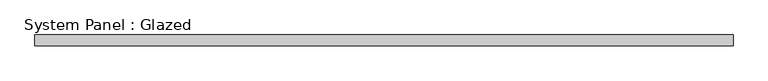
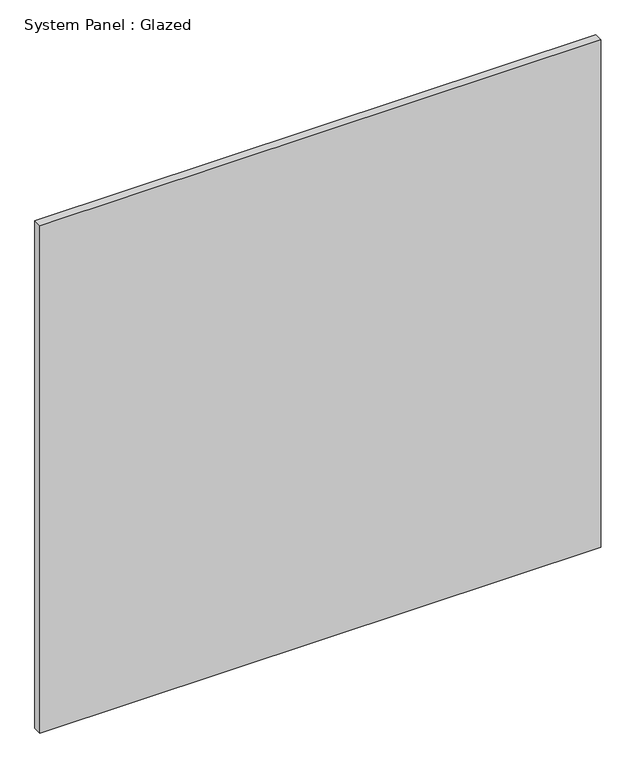
"""IFC4 building model written with IfcOpenShell, lengths in millimetres: plate geometry, System Panel : Glazed."""

from ifc_helpers import new_model, si_unit, origin, origin_with_axes, place, context, project, spatial, polyline, outline, extrude, source, transform, mapped, element, save


def system_panel_glazed_d780d238(model_context):
    return source(origin(), model_context, "Body", "SweptSolid", [
        extrude(outline(polyline([(810.0, 24.5), (-810.0, 24.5), (-810.0, 49.5), (810.0, 49.5), (810.0, 24.5)])), origin_with_axes(), (0.0, 0.0, 1.0), 1550.0),
    ])


if __name__ == "__main__":
    model = new_model("IFC4")
    model_context = context("Model", 3, world=origin())
    ifc_project = project(units=[si_unit("LENGTHUNIT", "METRE", prefix="MILLI")], contexts=[model_context])
    site = spatial("IfcSite", under=ifc_project)
    building = spatial("IfcBuilding", under=site)
    placement = place(None, origin())
    system_panel_glazed_shape = system_panel_glazed_d780d238(model_context)
    element("IfcPlate", 1, ObjectType="System Panel : Glazed", at=placement, inside=building, context=model_context, shape_type="MappedRepresentation", body=[
        mapped(system_panel_glazed_shape, transform((0.0, 0.0, 0.0), x_axis=(1.0, 0.0, 0.0), y_axis=(0.0, 1.0, 0.0), z_axis=(0.0, 0.0, 1.0))),
    ])
    save(model, "model.ifc")

# Revit data of these elements
# Element 1 (IfcPlate, "System Panel : Glazed")
#   Materials on its faces: "Glass"
# Materials
#   "Glass": class "Glass", colour RGB 0 128 192, transparency 0.9
